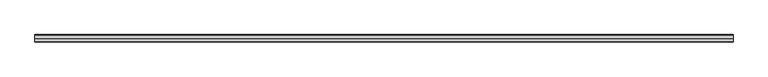
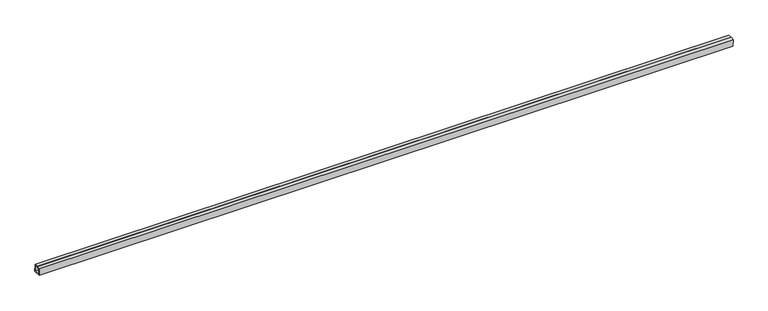
"""IFC4 building model written with IfcOpenShell, lengths in millimetres: proxy geometry, Inner panel:Inner panel:1:Inner panel:1 : Inner panel:Inner panel:300324:2:Inner panel:1:Inner panel:1 : Inner panel:Inner panel:300324:2 : Inner panel:Inner panel:1:Inner panel:1 : Inner panel:Inner panel:300324:300043:8 : Inner panel:Inner panel:1:Inner panel:1 : Inner panel:Inner panel:300324:2:Inner panel:1:Inner panel:1 : Inner panel:Inner panel:300324:2 : Inner panel:Inner panel:1:Inner panel:1 : Inner panel:Inner panel:300324:300043:308120."""

from ifc_helpers import new_model, si_unit, frame, origin, place, context, project, spatial, polyline, outline, extrude, source, transform, mapped, element, save


def generic_models_66b269a2(model_context):
    return source(origin(), model_context, "Body", "SweptSolid", [
        extrude(outline(polyline([(-576655.6949211, 4047.6065374), (-576637.4544979, 4048.3665551), (-576635.8683742, 4010.299585), (-576673.9353442, 4008.7134612), (-576675.521468, 4046.7804313), (-576657.2810448, 4047.540449), (-576657.1819121, 4045.1612633), (-576673.0431496, 4044.5003784), (-576671.6552914, 4011.1917796), (-576638.3466925, 4012.5796379), (-576639.7345508, 4045.8882367), (-576655.5957883, 4045.2273518), (-576655.6949211, 4047.6065374)])), frame((593141.1867239, 0.0, 0.0), z_axis=(1.0, 0.0, 0.0), x_axis=(0.0, 1.0, 0.0)), (0.0, 0.0, 1.0), 3657.6),
    ])


if __name__ == "__main__":
    model = new_model("IFC4")
    model_context = context("Model", 3, world=origin())
    ifc_project = project(units=[si_unit("LENGTHUNIT", "METRE", prefix="MILLI")], contexts=[model_context])
    site = spatial("IfcSite", under=ifc_project)
    building = spatial("IfcBuilding", under=site)
    placement = place(None, origin())
    generic_models_shape = generic_models_66b269a2(model_context)
    element("IfcBuildingElementProxy", 1, Name="Inner panel:Inner panel:1:Inner panel:1 : Inner panel:Inner panel:300324:2:Inner panel:1:Inner panel:1 : Inner panel:Inner panel:300324:2 : Inner panel:Inner panel:1:Inner panel:1 : Inner panel:Inner panel:300324:300043:8 : Inner panel:Inner panel:1:Inner panel:1 : Inner panel:Inner panel:300324:2:Inner panel:1:Inner panel:1 : Inner panel:Inner panel:300324:2 : Inner panel:Inner panel:1:Inner panel:1 : Inner panel:Inner panel:300324:300043:308120", ObjectType="Inner panel:Inner panel:1:Inner panel:1 : Inner panel:Inner panel:300324:2:Inner panel:1:Inner panel:1 : Inner panel:Inner panel:300324:2 : Inner panel:Inner panel:1:Inner panel:1 : Inner panel:Inner panel:300324:300043:8 : Inner panel:Inner panel:1:Inner panel:1 : Inner panel:Inner panel:300324:2:Inner panel:1:Inner panel:1 : Inner panel:Inner panel:300324:2 : Inner panel:Inner panel:1:Inner panel:1 : Inner panel:Inner panel:300324:300043:308120", at=placement, inside=building, context=model_context, shape_type="MappedRepresentation", body=[
        mapped(generic_models_shape, transform((0.0, 0.0, 0.0), x_axis=(1.0, 0.0, 0.0), y_axis=(0.0, 1.0, 0.0), z_axis=(0.0, 0.0, 1.0))),
    ])
    save(model, "model.ifc")

# Revit data of these elements
# Type "Inner panel:Inner panel:1:Inner panel:1 : Inner panel:Inner panel:300324:2:Inner panel:1:Inner panel:1 : Inner panel:Inner panel:300324:2 : Inner panel:Inner panel:1:Inner panel:1 : Inner panel:Inner panel:300324:300043:8 : Inner panel:Inner panel:1:Inner panel:1 : Inner panel:Inner panel:300324:2:Inner panel:1:Inner panel:1 : Inner panel:Inner panel:300324:2 : Inner panel:Inner panel:1:Inner panel:1 : Inner panel:Inner panel:300324:300043:308120"
#   NameOverride = "Inner panel:Inner panel:1:Inner panel:1 : Inner panel:Inner panel:300324:2:Inner panel:1:Inner panel:1 : Inner panel:Inner panel:300324:2 : Inner panel:Inner panel:1:Inner panel:1 : Inner panel:Inner panel:300324:300043:308120"
#   ObjectTypeOverride = "Inner panel:1:Inner panel:1 : Inner panel:Inner panel:300324:2 : Inner panel:Inner panel:1:Inner panel:1 : Inner panel:Inner panel:300324:300043"
#   Reference = "Inner panel"
#   Tag = "308120"
# Element 1 (IfcBuildingElementProxy, "Inner panel:Inner panel:1:Inner panel:1 : Inner panel:Inner panel:300324:2:Inner panel:1:Inner panel:1 : Inner panel:Inner panel:300324:2 : Inner panel:Inner panel:1:Inner panel:1 : Inner panel:Inner panel:300324:300043:8 : Inner panel:Inner panel:1:Inner panel:1 : Inner panel:Inner panel:300324:2:Inner panel:1:Inner panel:1 : Inner panel:Inner panel:300324:2 : Inner panel:Inner panel:1:Inner panel:1 : Inner panel:Inner panel:300324:300043:308120")
#   Materials on its faces: "1 1/2\" X 1 1/2\" SPLIT-SEAM SQUARE TUBING (~24\" CANTILEVER FROM C.L. OF GLULAM)"
# Materials
#   "1 1/2\" X 1 1/2\" SPLIT-SEAM SQUARE TUBING (~24\" CANTILEVER FROM C.L. OF GLULAM)": class "Unassigned", colour RGB 202 201 200, transparency 0, Cost = 0
